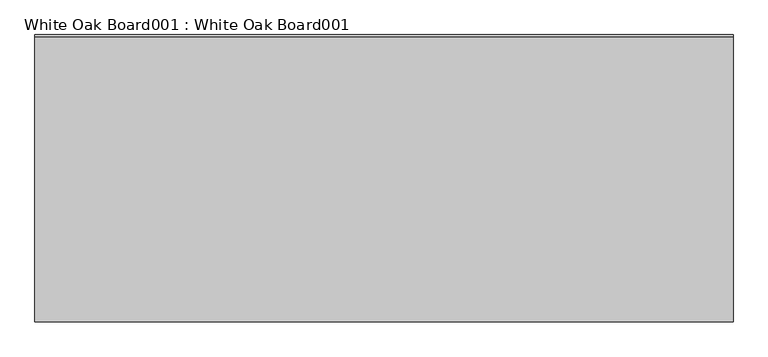
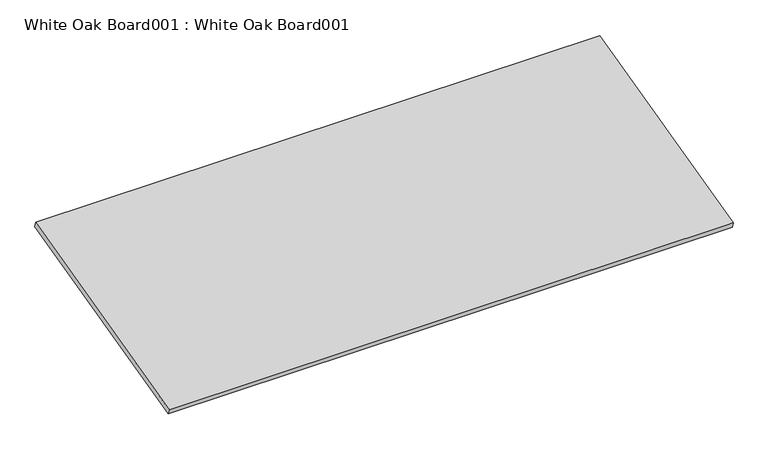
"""IFC4 building model written with IfcOpenShell, lengths in millimetres: proxy geometry, White Oak Board001 : White Oak Board001."""

from ifc_helpers import new_model, si_unit, frame, origin, place, context, project, spatial, polyline, outline, extrude, source, transform, mapped, element, save


def white_oak_board001_white_oak_board001_16393ac1(model_context):
    return source(origin(), model_context, "Body", "SweptSolid", [
        extrude(outline(polyline([(0.0, -844.55), (0.0, 0.0), (2000.25, 0.0), (2000.25, -844.55), (0.0, -844.55)])), frame((12382.7678845, -4420.1433685, 42614.5912441), z_axis=(0.0, -0.24292009113323607, 0.9700463026700428), x_axis=(1.0, 0.0, 0.0)), (0.0, 0.0, 1.0), 19.05),
    ])


if __name__ == "__main__":
    model = new_model("IFC4")
    model_context = context("Model", 3, world=origin())
    ifc_project = project(units=[si_unit("LENGTHUNIT", "METRE", prefix="MILLI")], contexts=[model_context])
    site = spatial("IfcSite", under=ifc_project)
    building = spatial("IfcBuilding", under=site)
    placement = place(None, origin())
    white_oak_board001_white_oak_board001_shape = white_oak_board001_white_oak_board001_16393ac1(model_context)
    element("IfcBuildingElementProxy", 1, Name="White Oak Board001 : White Oak Board001", ObjectType="White Oak Board001 : White Oak Board001", at=placement, inside=building, context=model_context, shape_type="MappedRepresentation", body=[
        mapped(white_oak_board001_white_oak_board001_shape, transform((0.0, 0.0, 0.0), x_axis=(1.0, 0.0, 0.0), y_axis=(0.0, 1.0, 0.0), z_axis=(0.0, 0.0, 1.0))),
    ])
    save(model, "model.ifc")

# Revit data of these elements
# Type "White Oak Board001 : White Oak Board001"
#   NameOverride = "White Oak Board001"
# Element 1 (IfcBuildingElementProxy, "White Oak Board001 : White Oak Board001")
#   Materials on its faces: "WHITE OAK (SPEC T.B.D.) OVER BUILDING WRAP"
# Materials
#   "WHITE OAK (SPEC T.B.D.) OVER BUILDING WRAP": class "Unassigned", colour RGB 227 188 136, transparency 0, Cost = 0
